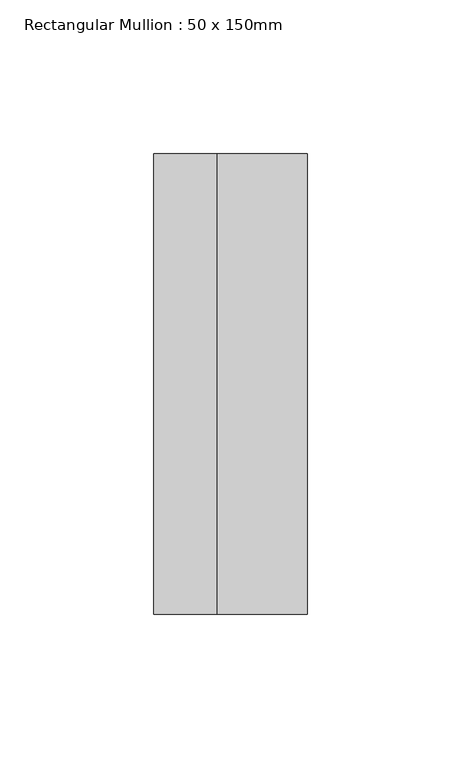
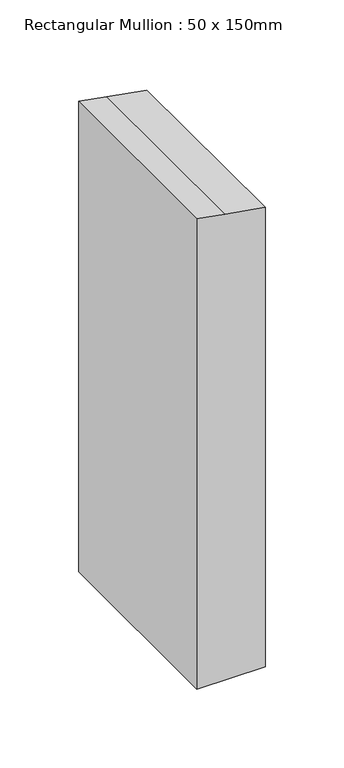
"""IFC4 building model written with IfcOpenShell, lengths in millimetres: member geometry, Rectangular Mullion : 50 x 150mm."""

import ifcopenshell
import ifcopenshell.guid

model = None  # the IFC model being written
_history = None  # IfcOwnerHistory: only IFC2X3 demands one
_inside = {}  # id of a spatial element -> (the spatial element, [elements in it])
_under = {}  # id of a project, library or spatial element -> (it, [spatial elements below it])
_declared = {}  # id of a project -> (the project, [libraries it declares])
_typed = {}  # id of a type object -> (the type object, [elements of that type])
_made_of = {}  # id of a material, layer set ... -> (it, [elements and type objects made of it])


def new_model(schema):
    """Start an empty IFC model of exactly this schema.

    Asked for "IFC4X3", IfcOpenShell would pick the latest addendum, in which some entities
    have other attributes; the version numbers below select the first issue.
    IFC2X3 requires an IfcOwnerHistory on every rooted entity: one is made here for all.
    """
    global model, _history
    if schema == "IFC4X3":
        model = ifcopenshell.file(schema_version=(4, 3, 0, 0))
    else:
        model = ifcopenshell.file(schema=schema)
    _inside.clear()
    _under.clear()
    _declared.clear()
    _typed.clear()
    _made_of.clear()
    _history = None
    if model.schema == "IFC2X3":
        org = make("IfcOrganization", Name="unknown")
        user = make(
            "IfcPersonAndOrganization",
            ThePerson=make("IfcPerson", FamilyName="unknown"),
            TheOrganization=org,
        )
        app = make(
            "IfcApplication",
            ApplicationDeveloper=org,
            Version="unknown",
            ApplicationFullName="unknown",
            ApplicationIdentifier="unknown",
        )
        _history = make(
            "IfcOwnerHistory",
            OwningUser=user,
            OwningApplication=app,
            ChangeAction="ADDED",
            CreationDate=0,
        )
    return model


def make(cls, **values):
    """One entity of the class cls with the attributes given. An attribute that is None is left unset."""
    return model.create_entity(
        cls, **{name: value for name, value in values.items() if value is not None}
    )


def rooted(cls, **values):
    """An entity with a GlobalId (a new one), such as an element, a storey or a relation."""
    return make(cls, GlobalId=ifcopenshell.guid.new(), OwnerHistory=_history, **values)


def si_unit(unit_type, name, prefix=None):
    """IfcSIUnit, for example si_unit("LENGTHUNIT", "METRE", prefix="MILLI")."""
    return make("IfcSIUnit", UnitType=unit_type, Prefix=prefix, Name=name)


def assignment(units):
    """IfcUnitAssignment: the units of a project."""
    return None if units is None else make("IfcUnitAssignment", Units=units)


def point(xyz):
    """IfcCartesianPoint."""
    return None if xyz is None else make("IfcCartesianPoint", Coordinates=xyz)


def direction(xyz):
    """IfcDirection."""
    return None if xyz is None else make("IfcDirection", DirectionRatios=xyz)


def frame(location, z_axis=None, x_axis=None):
    """IfcAxis2Placement3D, a coordinate frame: its origin and axes. An axis left out is left unset."""
    return make(
        "IfcAxis2Placement3D",
        Location=point(location),
        Axis=direction(z_axis),
        RefDirection=direction(x_axis),
    )


def origin():
    """The frame at (0, 0, 0) with its axes left unset."""
    return frame((0.0, 0.0, 0.0))


def place(relative_to, where):
    """IfcLocalPlacement: puts the frame where relative to a parent placement (None: the world)."""
    return make(
        "IfcLocalPlacement", PlacementRelTo=relative_to, RelativePlacement=where
    )


def context(
    kind, dimensions, precision=None, world=None, true_north=None, identifier=None
):
    """IfcGeometricRepresentationContext, for example the 3D "Model" context."""
    return make(
        "IfcGeometricRepresentationContext",
        ContextIdentifier=identifier,
        ContextType=kind,
        CoordinateSpaceDimension=dimensions,
        Precision=precision,
        WorldCoordinateSystem=world,
        TrueNorth=true_north,
    )


def project(units=None, contexts=None):
    """IfcProject with its units and contexts."""
    return rooted(
        "IfcProject",
        Name="project",
        RepresentationContexts=contexts,
        UnitsInContext=assignment(units),
    )


def spatial(cls, under=None, at=None, **own):
    """A site, building, storey or space (cls), placed at a placement, below another one or the project."""
    s = rooted(cls, ObjectPlacement=at, **own)
    if under is not None:
        _under.setdefault(under.id(), (under, []))[1].append(s)
    return s


def polyline(points):
    """IfcPolyline through the points."""
    return make("IfcPolyline", Points=[point(p) for p in points])


def outline(outer, holes=None, kind="AREA"):
    """IfcArbitraryClosedProfileDef: a profile drawn as a closed curve; with holes, ...WithVoids."""
    if holes is None:
        return make("IfcArbitraryClosedProfileDef", ProfileType=kind, OuterCurve=outer)
    return make(
        "IfcArbitraryProfileDefWithVoids",
        ProfileType=kind,
        OuterCurve=outer,
        InnerCurves=holes,
    )


def extrude(swept, where, along, depth):
    """IfcExtrudedAreaSolid: the profile swept, set in the frame where, extruded along a direction by depth."""
    return make(
        "IfcExtrudedAreaSolid",
        SweptArea=swept,
        Position=where,
        ExtrudedDirection=direction(along),
        Depth=depth,
    )


def shape(context_of_items, identifier, shape_type, items):
    """IfcShapeRepresentation: the items that make up one representation, for example the "Body"."""
    return make(
        "IfcShapeRepresentation",
        ContextOfItems=context_of_items,
        RepresentationIdentifier=identifier,
        RepresentationType=shape_type,
        Items=items,
    )


def source(mapping_origin, context_of_items, identifier, shape_type, items):
    """IfcRepresentationMap: a shape defined once, which mapped items show again and again."""
    return make(
        "IfcRepresentationMap",
        MappingOrigin=mapping_origin,
        MappedRepresentation=shape(context_of_items, identifier, shape_type, items),
    )


def transform(
    local_origin,
    x_axis=None,
    y_axis=None,
    z_axis=None,
    scale=None,
    scale2=None,
    scale3=None,
    uniform=True,
):
    """IfcCartesianTransformationOperator3D, or its non-uniform kind. x_axis, y_axis, z_axis: its Axis1, 2, 3."""
    if uniform:
        return make(
            "IfcCartesianTransformationOperator3D",
            Axis1=direction(x_axis),
            Axis2=direction(y_axis),
            LocalOrigin=point(local_origin),
            Scale=scale,
            Axis3=direction(z_axis),
        )
    return make(
        "IfcCartesianTransformationOperator3DnonUniform",
        Axis1=direction(x_axis),
        Axis2=direction(y_axis),
        LocalOrigin=point(local_origin),
        Scale=scale,
        Axis3=direction(z_axis),
        Scale2=scale2,
        Scale3=scale3,
    )


def mapped(mapping_source, mapping_target):
    """IfcMappedItem: shows the shape of a source again, moved by a transform."""
    return make(
        "IfcMappedItem", MappingSource=mapping_source, MappingTarget=mapping_target
    )


def made_of(thing, what):
    """Note that an element or type object is made of a material, layer set ...; save() writes the relation."""
    if what is not None:
        _made_of.setdefault(what.id(), (what, []))[1].append(thing)
    return thing


def element(
    cls,
    number,
    at=None,
    inside=None,
    cuts=None,
    type_object=None,
    material=None,
    context=None,
    identifier="Body",
    shape_type=None,
    held_by="IfcProductDefinitionShape",
    body=None,
    shapes=None,
    **own,
):
    """One element of the class cls, such as IfcWall. Its Tag is "e" and its number.

    at: its placement. inside: the storey or other place that contains it. cuts: it is an
    opening in that element (IfcRelVoidsElement). A single representation is given by context,
    identifier, shape_type and body (its items); several are given by shapes. held_by: the class
    of the entity that holds the representations. save() writes the other relations.
    """
    e = rooted(cls, Tag="e%d" % number, ObjectPlacement=at, **own)
    if body is not None:
        shapes = [shape(context, identifier, shape_type, body)]
    if shapes is not None:
        e.Representation = make(held_by, Representations=shapes)
    if inside is not None:
        _inside.setdefault(inside.id(), (inside, []))[1].append(e)
    if cuts is not None:
        rooted(
            "IfcRelVoidsElement", RelatingBuildingElement=cuts, RelatedOpeningElement=e
        )
    if type_object is not None:
        _typed.setdefault(type_object.id(), (type_object, []))[1].append(e)
    return made_of(e, material)


def aggregate(whole, parts):
    """IfcRelAggregates: a whole, such as a stair, and the parts it consists of."""
    return rooted("IfcRelAggregates", RelatingObject=whole, RelatedObjects=parts)


def save(model, path):
    """Write the relations noted so far, then the file.

    IfcRelAggregates (storeys below a building ...), IfcRelContainedInSpatialStructure (elements
    in a storey), IfcRelDefinesByType, IfcRelAssociatesMaterial and IfcRelDeclares: one each for
    every whole, place, type object, material and project.
    """
    for whole, parts in _under.values():
        aggregate(whole, parts)
    for where, things in _inside.values():
        rooted(
            "IfcRelContainedInSpatialStructure",
            RelatedElements=things,
            RelatingStructure=where,
        )
    for kind, things in _typed.values():
        rooted("IfcRelDefinesByType", RelatedObjects=things, RelatingType=kind)
    for what, things in _made_of.values():
        rooted("IfcRelAssociatesMaterial", RelatedObjects=things, RelatingMaterial=what)
    for by, libraries in _declared.values():
        rooted("IfcRelDeclares", RelatingContext=by, RelatedDefinitions=libraries)
    model.write(path)


def rectangular_mullion_50_x_150mm_bc448f9a(model_context):
    return source(origin(), model_context, "Body", "SweptSolid", [
        extrude(outline(polyline([(-4.7938398, 25.0), (0.3798062, -4.3412044), (4.0225092, -25.0), (-360.7536619, -25.0), (-360.7536619, 25.0), (-4.7938398, 25.0)])), frame((0.0, -75.0, 0.0), z_axis=(0.0, 1.0, 0.0), x_axis=(0.0, 0.0, 1.0)), (0.0, 0.0, 1.0), 150.0),
    ])


if __name__ == "__main__":
    model = new_model("IFC4")
    model_context = context("Model", 3, world=origin())
    ifc_project = project(units=[si_unit("LENGTHUNIT", "METRE", prefix="MILLI")], contexts=[model_context])
    site = spatial("IfcSite", under=ifc_project)
    building = spatial("IfcBuilding", under=site)
    placement = place(None, origin())
    rectangular_mullion_50_x_150mm_shape = rectangular_mullion_50_x_150mm_bc448f9a(model_context)
    element("IfcMember", 1, ObjectType="Rectangular Mullion : 50 x 150mm", at=placement, inside=building, context=model_context, shape_type="MappedRepresentation", body=[
        mapped(rectangular_mullion_50_x_150mm_shape, transform((0.0, 0.0, 0.0), x_axis=(1.0, 0.0, 0.0), y_axis=(0.0, 1.0, 0.0), z_axis=(0.0, 0.0, 1.0))),
    ])
    save(model, "model.ifc")

# Revit data of these elements
# Type "Rectangular Mullion : 50 x 150mm"
#   built-in parameter 1007304 = 0.492126 (stored number, unit not read)
#   built-in parameter 1007301 = 0.082021 (stored number, unit not read)
#   built-in parameter 1007300 = 0.082021 (stored number, unit not read)
# Element 1 (IfcMember, "Rectangular Mullion : 50 x 150mm")
#   Materials on its faces: "Aluminium"
# Materials
#   "Aluminium": class "Metal", colour RGB 247 247 247, transparency 0, Description = "Aluminium 6061", Cost = 0
